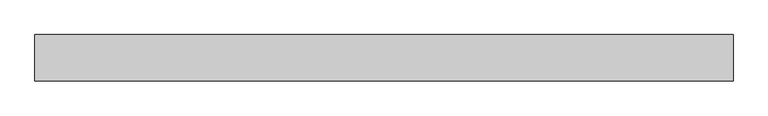
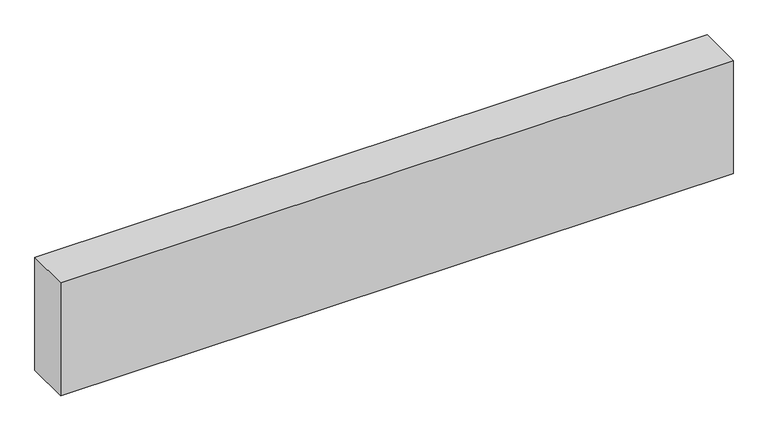
"""IFC4 building model written with IfcOpenShell, lengths in millimetres: proxy geometry, Structure004 554 : Structure004 554."""

from ifc_helpers import new_model, si_unit, frame, origin, place, context, project, spatial, polyline, outline, extrude, source, transform, mapped, element, save


def generic_models_b3b4ee5f(model_context):
    return source(origin(), model_context, "Body", "SweptSolid", [
        extrude(outline(polyline([(3694.2883192, 9587.4633229), (3694.2883192, 9720.8133229), (5694.2883192, 9720.8133229), (5694.2883192, 9587.4633229), (3694.2883192, 9587.4633229)])), frame((0.0, 0.0, 39757.096), z_axis=(0.0, 0.0, 1.0), x_axis=(1.0, 0.0, 0.0)), (0.0, 0.0, 1.0), 355.6),
    ])


if __name__ == "__main__":
    model = new_model("IFC4")
    model_context = context("Model", 3, world=origin())
    ifc_project = project(units=[si_unit("LENGTHUNIT", "METRE", prefix="MILLI")], contexts=[model_context])
    site = spatial("IfcSite", under=ifc_project)
    building = spatial("IfcBuilding", under=site)
    placement = place(None, origin())
    generic_models_shape = generic_models_b3b4ee5f(model_context)
    element("IfcBuildingElementProxy", 1, Name="Structure004 554 : Structure004 554", ObjectType="Structure004 554 : Structure004 554", at=placement, inside=building, context=model_context, shape_type="MappedRepresentation", body=[
        mapped(generic_models_shape, transform((0.0, 0.0, 0.0), x_axis=(1.0, 0.0, 0.0), y_axis=(0.0, 1.0, 0.0), z_axis=(0.0, 0.0, 1.0))),
    ])
    save(model, "model.ifc")

# Revit data of these elements
# Type "Structure004 554 : Structure004 554"
#   NameOverride = "Structure004"
# Element 1 (IfcBuildingElementProxy, "Structure004 554 : Structure004 554")
#   Materials on its faces: "STRUCTURAL MEMBER (SEE STRUCTURAL DWGS)"
# Materials
#   "STRUCTURAL MEMBER (SEE STRUCTURAL DWGS)": class "Unassigned", colour RGB 176 134 95, transparency 0, Cost = 0
